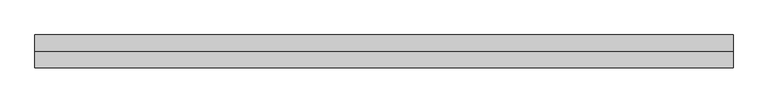
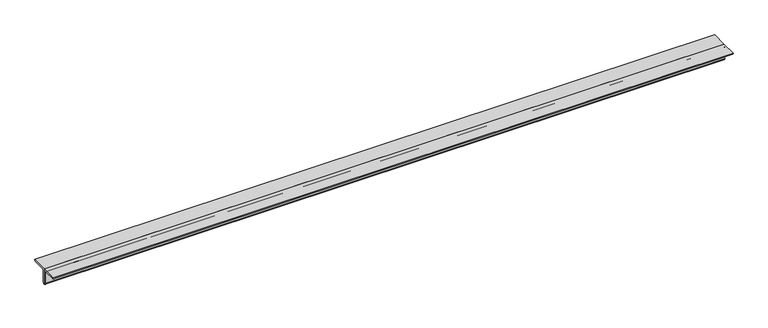
"""IFC4 building model written with IfcOpenShell, lengths in millimetres: member geometry, Steel Framing_2Ls_KS : H_SB_AR_S02_2Ls-100x100x10_VBR1."""

import ifcopenshell
import ifcopenshell.guid

model = None  # the IFC model being written
_history = None  # IfcOwnerHistory: only IFC2X3 demands one
_inside = {}  # id of a spatial element -> (the spatial element, [elements in it])
_under = {}  # id of a project, library or spatial element -> (it, [spatial elements below it])
_declared = {}  # id of a project -> (the project, [libraries it declares])
_typed = {}  # id of a type object -> (the type object, [elements of that type])
_made_of = {}  # id of a material, layer set ... -> (it, [elements and type objects made of it])


def new_model(schema):
    """Start an empty IFC model of exactly this schema.

    Asked for "IFC4X3", IfcOpenShell would pick the latest addendum, in which some entities
    have other attributes; the version numbers below select the first issue.
    IFC2X3 requires an IfcOwnerHistory on every rooted entity: one is made here for all.
    """
    global model, _history
    if schema == "IFC4X3":
        model = ifcopenshell.file(schema_version=(4, 3, 0, 0))
    else:
        model = ifcopenshell.file(schema=schema)
    _inside.clear()
    _under.clear()
    _declared.clear()
    _typed.clear()
    _made_of.clear()
    _history = None
    if model.schema == "IFC2X3":
        org = make("IfcOrganization", Name="unknown")
        user = make(
            "IfcPersonAndOrganization",
            ThePerson=make("IfcPerson", FamilyName="unknown"),
            TheOrganization=org,
        )
        app = make(
            "IfcApplication",
            ApplicationDeveloper=org,
            Version="unknown",
            ApplicationFullName="unknown",
            ApplicationIdentifier="unknown",
        )
        _history = make(
            "IfcOwnerHistory",
            OwningUser=user,
            OwningApplication=app,
            ChangeAction="ADDED",
            CreationDate=0,
        )
    return model


def make(cls, **values):
    """One entity of the class cls with the attributes given. An attribute that is None is left unset."""
    return model.create_entity(
        cls, **{name: value for name, value in values.items() if value is not None}
    )


def rooted(cls, **values):
    """An entity with a GlobalId (a new one), such as an element, a storey or a relation."""
    return make(cls, GlobalId=ifcopenshell.guid.new(), OwnerHistory=_history, **values)


def si_unit(unit_type, name, prefix=None):
    """IfcSIUnit, for example si_unit("LENGTHUNIT", "METRE", prefix="MILLI")."""
    return make("IfcSIUnit", UnitType=unit_type, Prefix=prefix, Name=name)


def assignment(units):
    """IfcUnitAssignment: the units of a project."""
    return None if units is None else make("IfcUnitAssignment", Units=units)


def point(xyz):
    """IfcCartesianPoint."""
    return None if xyz is None else make("IfcCartesianPoint", Coordinates=xyz)


def direction(xyz):
    """IfcDirection."""
    return None if xyz is None else make("IfcDirection", DirectionRatios=xyz)


def frame(location, z_axis=None, x_axis=None):
    """IfcAxis2Placement3D, a coordinate frame: its origin and axes. An axis left out is left unset."""
    return make(
        "IfcAxis2Placement3D",
        Location=point(location),
        Axis=direction(z_axis),
        RefDirection=direction(x_axis),
    )


def frame_2d(location, x_axis=None):
    """IfcAxis2Placement2D, a coordinate frame in the plane: its origin and x axis."""
    return make(
        "IfcAxis2Placement2D", Location=point(location), RefDirection=direction(x_axis)
    )


def origin():
    """The frame at (0, 0, 0) with its axes left unset."""
    return frame((0.0, 0.0, 0.0))


def place(relative_to, where):
    """IfcLocalPlacement: puts the frame where relative to a parent placement (None: the world)."""
    return make(
        "IfcLocalPlacement", PlacementRelTo=relative_to, RelativePlacement=where
    )


def context(
    kind, dimensions, precision=None, world=None, true_north=None, identifier=None
):
    """IfcGeometricRepresentationContext, for example the 3D "Model" context."""
    return make(
        "IfcGeometricRepresentationContext",
        ContextIdentifier=identifier,
        ContextType=kind,
        CoordinateSpaceDimension=dimensions,
        Precision=precision,
        WorldCoordinateSystem=world,
        TrueNorth=true_north,
    )


def project(units=None, contexts=None):
    """IfcProject with its units and contexts."""
    return rooted(
        "IfcProject",
        Name="project",
        RepresentationContexts=contexts,
        UnitsInContext=assignment(units),
    )


def spatial(cls, under=None, at=None, **own):
    """A site, building, storey or space (cls), placed at a placement, below another one or the project."""
    s = rooted(cls, ObjectPlacement=at, **own)
    if under is not None:
        _under.setdefault(under.id(), (under, []))[1].append(s)
    return s


def polyline(points):
    """IfcPolyline through the points."""
    return make("IfcPolyline", Points=[point(p) for p in points])


def circle_curve(where, radius):
    """IfcCircle in the frame where."""
    return make("IfcCircle", Position=where, Radius=radius)


def trimmed(basis, trim1, trim2, sense, master):
    """IfcTrimmedCurve: the piece of a basis curve between two trims."""
    return make(
        "IfcTrimmedCurve",
        BasisCurve=basis,
        Trim1=trim1,
        Trim2=trim2,
        SenseAgreement=sense,
        MasterRepresentation=master,
    )


def segment(curve, same_sense, transition):
    """IfcCompositeCurveSegment."""
    return make(
        "IfcCompositeCurveSegment",
        Transition=transition,
        SameSense=same_sense,
        ParentCurve=curve,
    )


def composite_curve(segments, self_intersect=None):
    """IfcCompositeCurve: segments joined end to end."""
    return make("IfcCompositeCurve", Segments=segments, SelfIntersect=self_intersect)


def outline(outer, holes=None, kind="AREA"):
    """IfcArbitraryClosedProfileDef: a profile drawn as a closed curve; with holes, ...WithVoids."""
    if holes is None:
        return make("IfcArbitraryClosedProfileDef", ProfileType=kind, OuterCurve=outer)
    return make(
        "IfcArbitraryProfileDefWithVoids",
        ProfileType=kind,
        OuterCurve=outer,
        InnerCurves=holes,
    )


def extrude(swept, where, along, depth):
    """IfcExtrudedAreaSolid: the profile swept, set in the frame where, extruded along a direction by depth."""
    return make(
        "IfcExtrudedAreaSolid",
        SweptArea=swept,
        Position=where,
        ExtrudedDirection=direction(along),
        Depth=depth,
    )


def shape(context_of_items, identifier, shape_type, items):
    """IfcShapeRepresentation: the items that make up one representation, for example the "Body"."""
    return make(
        "IfcShapeRepresentation",
        ContextOfItems=context_of_items,
        RepresentationIdentifier=identifier,
        RepresentationType=shape_type,
        Items=items,
    )


def source(mapping_origin, context_of_items, identifier, shape_type, items):
    """IfcRepresentationMap: a shape defined once, which mapped items show again and again."""
    return make(
        "IfcRepresentationMap",
        MappingOrigin=mapping_origin,
        MappedRepresentation=shape(context_of_items, identifier, shape_type, items),
    )


def transform(
    local_origin,
    x_axis=None,
    y_axis=None,
    z_axis=None,
    scale=None,
    scale2=None,
    scale3=None,
    uniform=True,
):
    """IfcCartesianTransformationOperator3D, or its non-uniform kind. x_axis, y_axis, z_axis: its Axis1, 2, 3."""
    if uniform:
        return make(
            "IfcCartesianTransformationOperator3D",
            Axis1=direction(x_axis),
            Axis2=direction(y_axis),
            LocalOrigin=point(local_origin),
            Scale=scale,
            Axis3=direction(z_axis),
        )
    return make(
        "IfcCartesianTransformationOperator3DnonUniform",
        Axis1=direction(x_axis),
        Axis2=direction(y_axis),
        LocalOrigin=point(local_origin),
        Scale=scale,
        Axis3=direction(z_axis),
        Scale2=scale2,
        Scale3=scale3,
    )


def mapped(mapping_source, mapping_target):
    """IfcMappedItem: shows the shape of a source again, moved by a transform."""
    return make(
        "IfcMappedItem", MappingSource=mapping_source, MappingTarget=mapping_target
    )


def made_of(thing, what):
    """Note that an element or type object is made of a material, layer set ...; save() writes the relation."""
    if what is not None:
        _made_of.setdefault(what.id(), (what, []))[1].append(thing)
    return thing


def element(
    cls,
    number,
    at=None,
    inside=None,
    cuts=None,
    type_object=None,
    material=None,
    context=None,
    identifier="Body",
    shape_type=None,
    held_by="IfcProductDefinitionShape",
    body=None,
    shapes=None,
    **own,
):
    """One element of the class cls, such as IfcWall. Its Tag is "e" and its number.

    at: its placement. inside: the storey or other place that contains it. cuts: it is an
    opening in that element (IfcRelVoidsElement). A single representation is given by context,
    identifier, shape_type and body (its items); several are given by shapes. held_by: the class
    of the entity that holds the representations. save() writes the other relations.
    """
    e = rooted(cls, Tag="e%d" % number, ObjectPlacement=at, **own)
    if body is not None:
        shapes = [shape(context, identifier, shape_type, body)]
    if shapes is not None:
        e.Representation = make(held_by, Representations=shapes)
    if inside is not None:
        _inside.setdefault(inside.id(), (inside, []))[1].append(e)
    if cuts is not None:
        rooted(
            "IfcRelVoidsElement", RelatingBuildingElement=cuts, RelatedOpeningElement=e
        )
    if type_object is not None:
        _typed.setdefault(type_object.id(), (type_object, []))[1].append(e)
    return made_of(e, material)


def aggregate(whole, parts):
    """IfcRelAggregates: a whole, such as a stair, and the parts it consists of."""
    return rooted("IfcRelAggregates", RelatingObject=whole, RelatedObjects=parts)


def save(model, path):
    """Write the relations noted so far, then the file.

    IfcRelAggregates (storeys below a building ...), IfcRelContainedInSpatialStructure (elements
    in a storey), IfcRelDefinesByType, IfcRelAssociatesMaterial and IfcRelDeclares: one each for
    every whole, place, type object, material and project.
    """
    for whole, parts in _under.values():
        aggregate(whole, parts)
    for where, things in _inside.values():
        rooted(
            "IfcRelContainedInSpatialStructure",
            RelatedElements=things,
            RelatingStructure=where,
        )
    for kind, things in _typed.values():
        rooted("IfcRelDefinesByType", RelatedObjects=things, RelatingType=kind)
    for what, things in _made_of.values():
        rooted("IfcRelAssociatesMaterial", RelatedObjects=things, RelatingMaterial=what)
    for by, libraries in _declared.values():
        rooted("IfcRelDeclares", RelatingContext=by, RelatedDefinitions=libraries)
    model.write(path)


def member_c612666d(model_context):
    return source(origin(), model_context, "Body", "SweptSolid", [
        extrude(outline(composite_curve([segment(polyline([(0.0, 28.2), (100.0, 28.2)]), True, "CONTINUOUS"), segment(trimmed(circle_curve(frame_2d((90.0, 28.2)), 10.0), [point((100.0, 28.2))], [point((90.0, 18.2))], False, "CARTESIAN"), True, "CONTINUOUS"), segment(polyline([(90.0, 18.2), (20.0, 18.2)]), True, "CONTINUOUS"), segment(trimmed(circle_curve(frame_2d((20.0, 8.2)), 10.0), [point((20.0, 18.2))], [point((10.0, 8.2))], True, "CARTESIAN"), True, "CONTINUOUS"), segment(polyline([(10.0, 8.2), (10.0, -61.8)]), True, "CONTINUOUS"), segment(trimmed(circle_curve(frame_2d((0.0, -61.8)), 10.0), [point((10.0, -61.8))], [point((0.0, -71.8))], False, "CARTESIAN"), True, "CONTINUOUS"), segment(polyline([(0.0, -71.8), (0.0, 28.2)]), True, "CONTINUOUS")], self_intersect=False)), frame((-2041.6751257, 0.0, 0.0), z_axis=(1.0, 0.0, 0.0), x_axis=(0.0, 1.0, 0.0)), (0.0, 0.0, 1.0), 4232.1149008),
        extrude(outline(composite_curve([segment(polyline([(0.0, 28.2), (0.0, -71.8)]), True, "CONTINUOUS"), segment(trimmed(circle_curve(frame_2d((0.0, -61.8)), 10.0), [point((0.0, -71.8))], [point((-10.0, -61.8))], False, "CARTESIAN"), True, "CONTINUOUS"), segment(polyline([(-10.0, -61.8), (-10.0, 8.2)]), True, "CONTINUOUS"), segment(trimmed(circle_curve(frame_2d((-20.0, 8.2)), 10.0), [point((-10.0, 8.2))], [point((-20.0, 18.2))], True, "CARTESIAN"), True, "CONTINUOUS"), segment(polyline([(-20.0, 18.2), (-90.0, 18.2)]), True, "CONTINUOUS"), segment(trimmed(circle_curve(frame_2d((-90.0, 28.2)), 10.0), [point((-90.0, 18.2))], [point((-100.0, 28.2))], False, "CARTESIAN"), True, "CONTINUOUS"), segment(polyline([(-100.0, 28.2), (0.0, 28.2)]), True, "CONTINUOUS")], self_intersect=False)), frame((-2041.6751257, 0.0, 0.0), z_axis=(1.0, 0.0, 0.0), x_axis=(0.0, 1.0, 0.0)), (0.0, 0.0, 1.0), 4232.1149008),
    ])


if __name__ == "__main__":
    model = new_model("IFC4")
    model_context = context("Model", 3, world=origin())
    ifc_project = project(units=[si_unit("LENGTHUNIT", "METRE", prefix="MILLI")], contexts=[model_context])
    site = spatial("IfcSite", under=ifc_project)
    building = spatial("IfcBuilding", under=site)
    placement = place(None, origin())
    member_shape = member_c612666d(model_context)
    element("IfcMember", 1, ObjectType="Steel Framing_2Ls_KS : H_SB_AR_S02_2Ls-100x100x10_VBR1", at=placement, inside=building, context=model_context, shape_type="MappedRepresentation", body=[
        mapped(member_shape, transform((0.0, 0.0, 0.0), x_axis=(1.0, 0.0, 0.0), y_axis=(0.0, 1.0, 0.0), z_axis=(0.0, 0.0, 1.0))),
    ])
    save(model, "model.ifc")

# Revit data of these elements
# Type "Steel Framing_2Ls_KS : H_SB_AR_S02_2Ls-100x100x10_VBR1"
#   Type Comments = "MAIN"
#   Type Mark = "VBR1"
#   H_SectionID = "2Ls-100x100x10"
#   Assembly Code = "B10"
#   Legs = "LLBB"
#   H_Ratio for Additional Steel Plate = 0.2
#   W = 0
#   Perimeter = 0.80 m²/m
#   Nominal Weight = 29.80 kgf/m
#   Length [instance default] = 1524 mm
#   Space = 0 mm
#   b = 100 mm
#   d = 100 mm
#   t = 10 mm
#   y = 28.2 mm
#   A = 0.0038 m²
#   Structural Material [instance default] = Steel, 45-345
# Element 1 (IfcMember, "Steel Framing_2Ls_KS : H_SB_AR_S02_2Ls-100x100x10_VBR1")
#   Materials on its faces: "Steel, 45-345"
# Materials
#   "Steel, 45-345": class "Metal", colour RGB 189 187 185, transparency 0, Description = "Steel 345 MPa", Cost = 0
